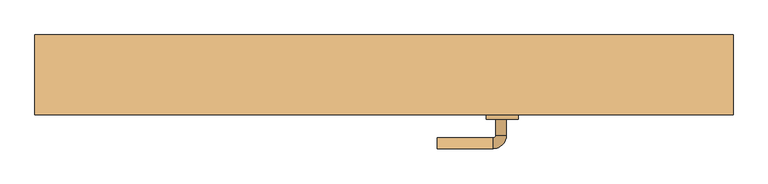
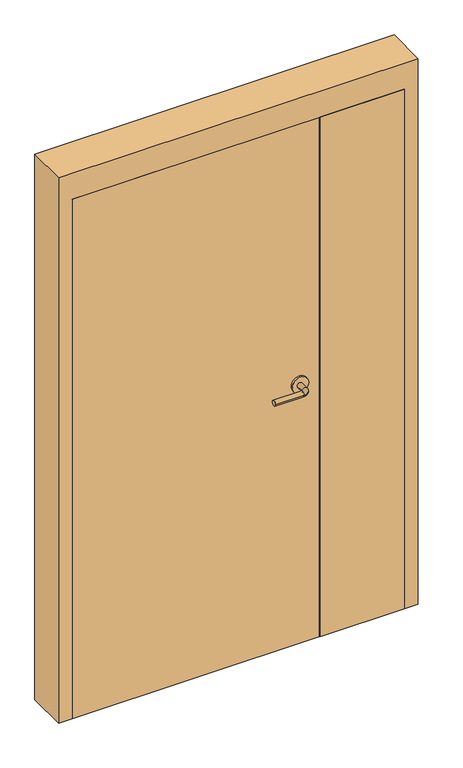
"""IFC4 building model written with IfcOpenShell, lengths in millimetres: door geometry, Дверь-Маятниковая-С полотнами разной ширины-Щитовая : 1310 x 2100 мм."""

from ifc_helpers import new_model, si_unit, point, frame, frame_2d, origin, origin_with_axes, place, context, project, spatial, polyline, circle_curve, ellipse_curve, trimmed, segment, composite_curve, outline, extrude, faceted_brep, source, transform, mapped, element, save
from ifc_brep_helpers import plane_surface, cylinder_surface, revolved_surface, advanced_brep


def door_cb375475(model_context):
    return source(origin(), model_context, "Body", "SolidModel", [
        advanced_brep(
        [(229.59375, -15.85, 1000.0), (209.59375, -15.85, 1000.0), (209.59375, 14.15, 1000.0), (229.59375, 14.15, 1000.0), (204.59375, 19.15, 1000.0), (204.59375, 39.15, 1000.0), (99.59375, 39.15, 1000.0), (99.59375, 19.15, 1000.0)],
        [
            (0, 1, circle_curve(frame((219.59375, -15.85, 1000.0), z_axis=(0.0, -1.0, 0.0), x_axis=(-1.0, 0.0, 0.0)), 10.0)),
            (1, 0, circle_curve(frame((219.59375, -15.85, 1000.0), z_axis=(0.0, -1.0, 0.0), x_axis=(-1.0, 0.0, 0.0)), 10.0)),
            (1, 2),
            (2, 3, circle_curve(frame((219.59375, 14.15, 1000.0), z_axis=(0.0, -1.0, 0.0), x_axis=(-1.0, 0.0, 0.0)), 10.0)),
            (3, 0),
            (3, 2, circle_curve(frame((219.59375, 14.15, 1000.0), z_axis=(0.0, -1.0, 0.0), x_axis=(-1.0, 0.0, 0.0)), 10.0)),
            (4, 5, circle_curve(frame((204.59375, 29.15, 1000.0), z_axis=(1.0, 0.0, 0.0), x_axis=(0.0, -1.0, 0.0)), 10.0)),
            (5, 3, circle_curve(frame((204.59375, 14.15, 1000.0), z_axis=(0.0, 0.0, -1.0), x_axis=(1.0, 0.0, 0.0)), 25.0)),
            (2, 4, circle_curve(frame((204.59375, 14.15, 1000.0), z_axis=(0.0, 0.0, 1.0), x_axis=(1.0, 0.0, 0.0)), 5.0)),
            (5, 4, circle_curve(frame((204.59375, 29.15, 1000.0), z_axis=(1.0, 0.0, 0.0), x_axis=(0.0, -1.0, 0.0)), 10.0)),
            (6, 7, circle_curve(frame((99.59375, 29.15, 1000.0), z_axis=(-1.0, 0.0, 0.0), x_axis=(0.0, -1.0, 0.0)), 10.0)),
            (7, 6, circle_curve(frame((99.59375, 29.15, 1000.0), z_axis=(-1.0, 0.0, 0.0), x_axis=(0.0, -1.0, 0.0)), 10.0)),
            (4, 7),
            (6, 5),
        ],
        [
            plane_surface(frame((219.59375, -15.85, 1000.0), z_axis=(0.0, -1.0, 0.0), x_axis=(0.0, 0.0, 1.0))),
            cylinder_surface(frame((219.59375, -15.85, 1000.0), z_axis=(0.0, -1.0, 0.0), x_axis=(-1.0, 0.0, 0.0)), 10.0),
            revolved_surface(trimmed(ellipse_curve(frame((219.59375, 14.15, 1000.0), z_axis=(0.0, 1.0, 0.0), x_axis=(-1.0, 0.0, 0.0)), 10.0, 10.0), [point((229.59375, 14.15, 1000.0))], [point((209.59375, 14.15, 1000.0))], True, "CARTESIAN"), (204.59375, 14.15, 1000.0), (0.0, 0.0, -1.0)),
            revolved_surface(trimmed(ellipse_curve(frame((219.59375, 14.15, 1000.0), z_axis=(0.0, 1.0, 0.0), x_axis=(-1.0, 0.0, 0.0)), 10.0, 10.0), [point((209.59375, 14.15, 1000.0))], [point((229.59375, 14.15, 1000.0))], True, "CARTESIAN"), (204.59375, 14.15, 1000.0), (0.0, 0.0, -1.0)),
            plane_surface(frame((99.59375, 29.15, 1000.0), z_axis=(-1.0, 0.0, 0.0), x_axis=(0.0, 0.0, 1.0))),
            cylinder_surface(frame((204.59375, 29.15, 1000.0), z_axis=(1.0, 0.0, 0.0), x_axis=(0.0, -1.0, 0.0)), 10.0),
        ],
        [
            (0, [[1, 2]]),
            (1, [[3, 4, 5, -2]]),
            (1, [[-5, 6, -3, -1]]),
            (2, [[7, 8, -4, 9]]),
            (3, [[10, -9, -6, -8]]),
            (4, [[11, 12]]),
            (5, [[13, -11, 14, -7]]),
            (5, [[-14, -12, -13, -10]]),
        ],
    ),
        extrude(outline(composite_curve([segment(trimmed(circle_curve(frame_2d((1000.0, 222.09375)), 30.0), [point((1000.0, 252.09375))], [point((1000.0, 192.09375))], False, "CARTESIAN"), True, "CONTINUOUS"), segment(trimmed(circle_curve(frame_2d((1000.0, 222.09375)), 30.0), [point((1000.0, 192.09375))], [point((1000.0, 252.09375))], False, "CARTESIAN"), True, "CONTINUOUS")], self_intersect=False)), frame((0.0, -23.85, 0.0), z_axis=(0.0, 1.0, 0.0), x_axis=(0.0, 0.0, 1.0)), (0.0, 0.0, 1.0), 8.0),
        advanced_brep(
        [(229.59375, -76.85, 1000.0), (209.59375, -76.85, 1000.0), (229.59375, -106.85, 1000.0), (209.59375, -106.85, 1000.0), (204.59375, -111.85, 1000.0), (204.59375, -131.85, 1000.0), (99.59375, -131.85, 1000.0), (99.59375, -111.85, 1000.0)],
        [
            (0, 1, circle_curve(frame((219.59375, -76.85, 1000.0), z_axis=(0.0, 1.0, 0.0), x_axis=(-1.0, 0.0, 0.0)), 10.0)),
            (1, 0, circle_curve(frame((219.59375, -76.85, 1000.0), z_axis=(0.0, 1.0, 0.0), x_axis=(-1.0, 0.0, 0.0)), 10.0)),
            (0, 2),
            (2, 3, circle_curve(frame((219.59375, -106.85, 1000.0), z_axis=(0.0, 1.0, 0.0), x_axis=(-1.0, 0.0, 0.0)), 10.0)),
            (3, 1),
            (3, 2, circle_curve(frame((219.59375, -106.85, 1000.0), z_axis=(0.0, 1.0, 0.0), x_axis=(-1.0, 0.0, 0.0)), 10.0)),
            (4, 3, circle_curve(frame((204.59375, -106.85, 1000.0), z_axis=(0.0, 0.0, 1.0), x_axis=(1.0, 0.0, 0.0)), 5.0)),
            (2, 5, circle_curve(frame((204.59375, -106.85, 1000.0), z_axis=(0.0, 0.0, -1.0), x_axis=(1.0, 0.0, 0.0)), 25.0)),
            (5, 4, circle_curve(frame((204.59375, -121.85, 1000.0), z_axis=(1.0, 0.0, 0.0), x_axis=(0.0, 1.0, 0.0)), 10.0)),
            (4, 5, circle_curve(frame((204.59375, -121.85, 1000.0), z_axis=(1.0, 0.0, 0.0), x_axis=(0.0, 1.0, 0.0)), 10.0)),
            (6, 7, circle_curve(frame((99.59375, -121.85, 1000.0), z_axis=(-1.0, 0.0, 0.0), x_axis=(0.0, 1.0, 0.0)), 10.0)),
            (7, 6, circle_curve(frame((99.59375, -121.85, 1000.0), z_axis=(-1.0, 0.0, 0.0), x_axis=(0.0, 1.0, 0.0)), 10.0)),
            (5, 6),
            (7, 4),
        ],
        [
            plane_surface(frame((219.59375, -76.85, 1000.0), z_axis=(0.0, 1.0, 0.0), x_axis=(0.0, 0.0, 1.0))),
            cylinder_surface(frame((219.59375, -76.85, 1000.0), z_axis=(0.0, 1.0, 0.0), x_axis=(-1.0, 0.0, 0.0)), 10.0),
            revolved_surface(trimmed(ellipse_curve(frame((219.59375, -106.85, 1000.0), z_axis=(0.0, 1.0, 0.0), x_axis=(-1.0, 0.0, 0.0)), 10.0, 10.0), [point((229.59375, -106.85, 1000.0))], [point((209.59375, -106.85, 1000.0))], True, "CARTESIAN"), (204.59375, -106.85, 1000.0), (0.0, 0.0, -1.0)),
            revolved_surface(trimmed(ellipse_curve(frame((219.59375, -106.85, 1000.0), z_axis=(0.0, 1.0, 0.0), x_axis=(-1.0, 0.0, 0.0)), 10.0, 10.0), [point((209.59375, -106.85, 1000.0))], [point((229.59375, -106.85, 1000.0))], True, "CARTESIAN"), (204.59375, -106.85, 1000.0), (0.0, 0.0, -1.0)),
            plane_surface(frame((99.59375, -121.85, 1000.0), z_axis=(-1.0, 0.0, 0.0), x_axis=(0.0, 0.0, 1.0))),
            cylinder_surface(frame((204.59375, -121.85, 1000.0), z_axis=(1.0, 0.0, 0.0), x_axis=(0.0, 1.0, 0.0)), 10.0),
        ],
        [
            (0, [[1, 2]]),
            (1, [[-1, 3, 4, 5]]),
            (1, [[-2, -5, 6, -3]]),
            (2, [[7, -4, 8, 9]]),
            (3, [[-8, -6, -7, 10]]),
            (4, [[11, 12]]),
            (5, [[-9, 13, -12, 14]]),
            (5, [[-10, -14, -11, -13]]),
        ],
    ),
        extrude(outline(composite_curve([segment(trimmed(circle_curve(frame_2d((1000.0, 222.09375)), 30.0), [point((1000.0, 252.09375))], [point((1000.0, 192.09375))], False, "CARTESIAN"), True, "CONTINUOUS"), segment(trimmed(circle_curve(frame_2d((1000.0, 222.09375)), 30.0), [point((1000.0, 192.09375))], [point((1000.0, 252.09375))], False, "CARTESIAN"), True, "CONTINUOUS")], self_intersect=False)), frame((0.0, -76.85, 0.0), z_axis=(0.0, 1.0, 0.0), x_axis=(0.0, 0.0, 1.0)), (0.0, 0.0, 1.0), 8.0),
        extrude(outline(polyline([(605.0, -23.85), (605.0, -68.85), (296.6, -68.85), (296.6, -23.85), (605.0, -23.85)])), origin_with_axes(), (0.0, 0.0, 1.0), 2000.0),
        faceted_brep([(605.0, -19.0875, 0.0), (589.125, -19.0875, 0.0), (589.125, 31.9375, 0.0), (605.0, 31.9375, 0.0), (605.0, 81.15, 0.0), (655.0, 81.15, 0.0), (655.0, -68.85, 0.0), (605.0, -68.85, 0.0), (605.0, -68.85, 2000.0), (605.0, -19.0875, 2000.0), (655.0, -68.85, 2100.0), (-655.0, -68.85, 2100.0), (-655.0, -68.85, 0.0), (-605.0, -68.85, 0.0), (-605.0, -68.85, 2000.0), (655.0, 81.15, 2100.0), (605.0, 81.15, 2000.0), (-605.0, 81.15, 2000.0), (-605.0, 81.15, 0.0), (-655.0, 81.15, 0.0), (-655.0, 81.15, 2100.0), (605.0, 31.9375, 2000.0), (589.125, 31.9375, 1984.125), (-589.125, 31.9375, 1984.125), (-589.125, 31.9375, 0.0), (-605.0, 31.9375, 0.0), (-605.0, 31.9375, 2000.0), (589.125, -19.0875, 1984.125), (-605.0, -19.0875, 2000.0), (-605.0, -19.0875, 0.0), (-589.125, -19.0875, 0.0), (-589.125, -19.0875, 1984.125)], [[[0, 1, 2, 3, 4, 5, 6, 7]], [[7, 8, 9, 0]], [[6, 10, 11, 12, 13, 14, 8, 7]], [[5, 15, 10, 6]], [[4, 16, 17, 18, 19, 20, 15, 5]], [[3, 21, 16, 4]], [[2, 22, 23, 24, 25, 26, 21, 3]], [[1, 27, 22, 2]], [[0, 9, 28, 29, 30, 31, 27, 1]], [[8, 14, 28, 9]], [[16, 21, 26, 17]], [[22, 27, 31, 23]], [[12, 19, 18, 25, 24, 30, 29, 13]], [[13, 29, 28, 14]], [[11, 20, 19, 12]], [[17, 26, 25, 18]], [[23, 31, 30, 24]], [[15, 20, 11, 10]]]),
        extrude(outline(polyline([(293.4, -23.85), (293.4, -68.85), (-605.0, -68.85), (-605.0, -23.85), (293.4, -23.85)])), origin_with_axes(), (0.0, 0.0, 1.0), 2000.0),
    ])


if __name__ == "__main__":
    model = new_model("IFC4")
    model_context = context("Model", 3, world=origin())
    ifc_project = project(units=[si_unit("LENGTHUNIT", "METRE", prefix="MILLI")], contexts=[model_context])
    site = spatial("IfcSite", under=ifc_project)
    building = spatial("IfcBuilding", under=site)
    placement = place(None, origin())
    door_shape = door_cb375475(model_context)
    element("IfcDoor", 1, ObjectType="Дверь-Маятниковая-С полотнами разной ширины-Щитовая : 1310 x 2100 мм", at=placement, inside=building, context=model_context, shape_type="MappedRepresentation", body=[
        mapped(door_shape, transform((0.0, 0.0, 0.0), x_axis=(1.0, 0.0, 0.0), y_axis=(0.0, 1.0, 0.0), z_axis=(0.0, 0.0, 1.0))),
    ])
    save(model, "model.ifc")

# Revit data of these elements
# Type "Дверь-Маятниковая-С полотнами разной ширины-Щитовая : 1310 x 2100 мм"
#   Type Mark = "150"
#   Assembly Code = "C1020300"
#   Analytic Construction = "Деревянный"
#   Ширина большой панели = 900 mm
#   W = 310 mm
#   Thickness = 45 mm
#   Thermal Resistance (R) = 0.455703 (m²·K)/W
#   Угол поворота [instance default] = 90°
#   Высота планки = 1000 mm
#   Rough Width [instance default] = 1310 mm
#   Rough Height [instance default] = 2100 mm
#   Высота проема в кирпичном каркасе [instance default] = 100 mm
#   Ширина проема в кирпичном каркасе [instance default] = 100 mm
#   Расчет вставки [instance default] = 105 mm
#   Кирпичная вставка [instance default] = 25 mm
#   Height = 2000 mm
#   Width = 1210 mm
#   Heat Transfer Coefficient (U) = 2.19465 W/(m²·K)
#   Глубина кирпичного каркаса = 150 mm
#   Кирпичный каркас [instance default] = yes
#   Каркас стены сухой кладки [instance default] = no
#   Материал панели = Древесина - Береза
#   Материал каркаса = Металл - Окрашенный - Серый 2
#   Материал дверной ручки = Алюминий
#   Visual Light Transmittance = 0
#   Solar Heat Gain Coefficient = 0
#   Wall Closure = (empty or 0)
#   Function = (empty or 0)
# Element 1 (IfcDoor, "Дверь-Маятниковая-С полотнами разной ширины-Щитовая : 1310 x 2100 мм")
#   Расчет вставки = 80 mm
#   Кирпичная вставка = 0 mm
#   Materials on its faces: "Алюминий", "Металл - Окрашенный - Серый 2", "Древесина - Береза"
# Materials
#   "Древесина - Береза": class "Древесина", colour RGB 166 116 52, transparency 0, Cost = 0
#   "Металл - Окрашенный - Серый 2": class "Краска", colour RGB 104 104 104, transparency 0, Cost = 0
#   "Алюминий": class "Металл", colour RGB 247 247 247, transparency 0
